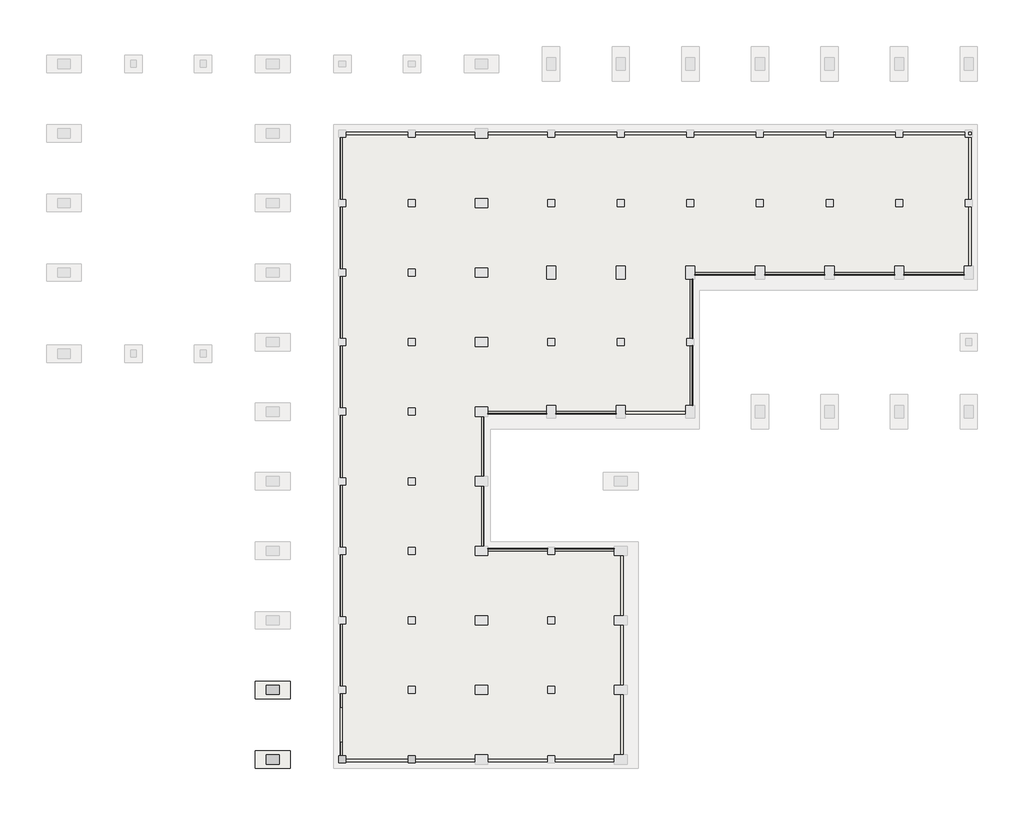
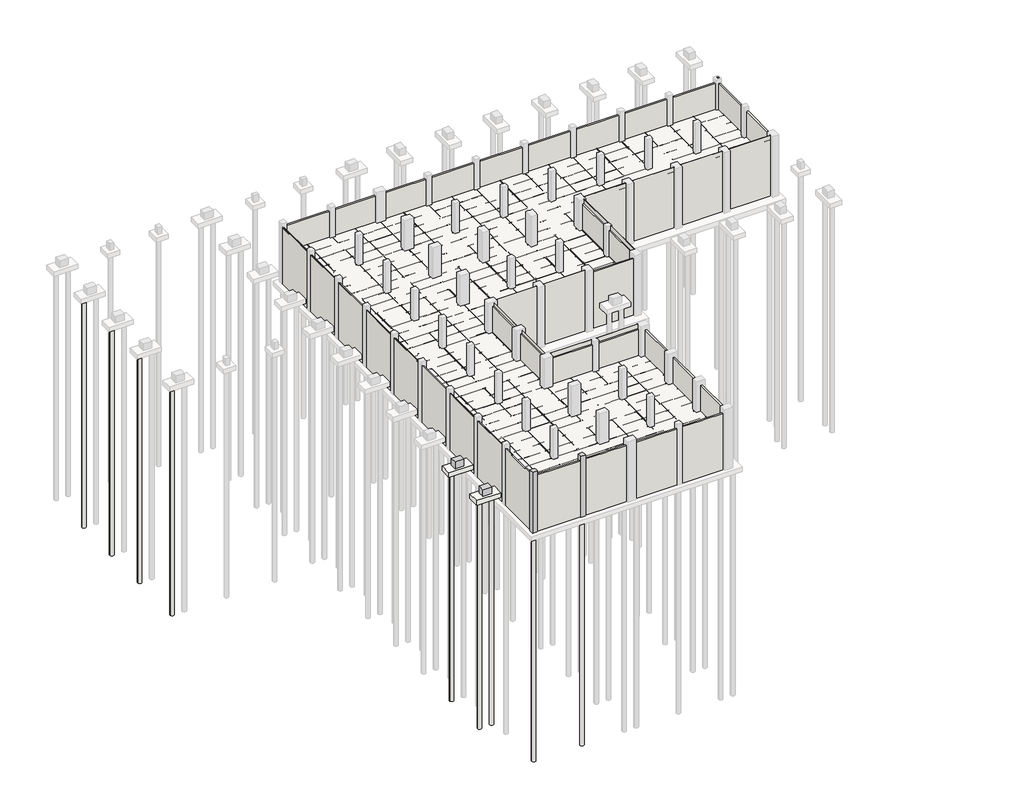
# Not in any storey, part 1 of 16: 12 slabs, 10 walls, 8 beams, 4 columns.
"""IFC4 building model written with IfcOpenShell, lengths in millimetres."""

import ifcopenshell
import ifcopenshell.guid

model = None  # the IFC model being written
_history = None  # IfcOwnerHistory: only IFC2X3 demands one
_inside = {}  # id of a spatial element -> (the spatial element, [elements in it])
_under = {}  # id of a project, library or spatial element -> (it, [spatial elements below it])
_declared = {}  # id of a project -> (the project, [libraries it declares])
_typed = {}  # id of a type object -> (the type object, [elements of that type])
_made_of = {}  # id of a material, layer set ... -> (it, [elements and type objects made of it])


def new_model(schema):
    """Start an empty IFC model of exactly this schema.

    Asked for "IFC4X3", IfcOpenShell would pick the latest addendum, in which some entities
    have other attributes; the version numbers below select the first issue.
    IFC2X3 requires an IfcOwnerHistory on every rooted entity: one is made here for all.
    """
    global model, _history
    if schema == "IFC4X3":
        model = ifcopenshell.file(schema_version=(4, 3, 0, 0))
    else:
        model = ifcopenshell.file(schema=schema)
    _inside.clear()
    _under.clear()
    _declared.clear()
    _typed.clear()
    _made_of.clear()
    _history = None
    if model.schema == "IFC2X3":
        org = make("IfcOrganization", Name="unknown")
        user = make(
            "IfcPersonAndOrganization",
            ThePerson=make("IfcPerson", FamilyName="unknown"),
            TheOrganization=org,
        )
        app = make(
            "IfcApplication",
            ApplicationDeveloper=org,
            Version="unknown",
            ApplicationFullName="unknown",
            ApplicationIdentifier="unknown",
        )
        _history = make(
            "IfcOwnerHistory",
            OwningUser=user,
            OwningApplication=app,
            ChangeAction="ADDED",
            CreationDate=0,
        )
    return model


def make(cls, **values):
    """One entity of the class cls with the attributes given. An attribute that is None is left unset."""
    return model.create_entity(
        cls, **{name: value for name, value in values.items() if value is not None}
    )


def rooted(cls, **values):
    """An entity with a GlobalId (a new one), such as an element, a storey or a relation."""
    return make(cls, GlobalId=ifcopenshell.guid.new(), OwnerHistory=_history, **values)


def si_unit(unit_type, name, prefix=None):
    """IfcSIUnit, for example si_unit("LENGTHUNIT", "METRE", prefix="MILLI")."""
    return make("IfcSIUnit", UnitType=unit_type, Prefix=prefix, Name=name)


def assignment(units):
    """IfcUnitAssignment: the units of a project."""
    return None if units is None else make("IfcUnitAssignment", Units=units)


def point(xyz):
    """IfcCartesianPoint."""
    return None if xyz is None else make("IfcCartesianPoint", Coordinates=xyz)


def direction(xyz):
    """IfcDirection."""
    return None if xyz is None else make("IfcDirection", DirectionRatios=xyz)


def frame(location, z_axis=None, x_axis=None):
    """IfcAxis2Placement3D, a coordinate frame: its origin and axes. An axis left out is left unset."""
    return make(
        "IfcAxis2Placement3D",
        Location=point(location),
        Axis=direction(z_axis),
        RefDirection=direction(x_axis),
    )


def frame_2d(location, x_axis=None):
    """IfcAxis2Placement2D, a coordinate frame in the plane: its origin and x axis."""
    return make(
        "IfcAxis2Placement2D", Location=point(location), RefDirection=direction(x_axis)
    )


def origin():
    """The frame at (0, 0, 0) with its axes left unset."""
    return frame((0.0, 0.0, 0.0))


def place(relative_to, where):
    """IfcLocalPlacement: puts the frame where relative to a parent placement (None: the world)."""
    return make(
        "IfcLocalPlacement", PlacementRelTo=relative_to, RelativePlacement=where
    )


def context(
    kind, dimensions, precision=None, world=None, true_north=None, identifier=None
):
    """IfcGeometricRepresentationContext, for example the 3D "Model" context."""
    return make(
        "IfcGeometricRepresentationContext",
        ContextIdentifier=identifier,
        ContextType=kind,
        CoordinateSpaceDimension=dimensions,
        Precision=precision,
        WorldCoordinateSystem=world,
        TrueNorth=true_north,
    )


def project(units=None, contexts=None):
    """IfcProject with its units and contexts."""
    return rooted(
        "IfcProject",
        Name="project",
        RepresentationContexts=contexts,
        UnitsInContext=assignment(units),
    )


def spatial(cls, under=None, at=None, **own):
    """A site, building, storey or space (cls), placed at a placement, below another one or the project."""
    s = rooted(cls, ObjectPlacement=at, **own)
    if under is not None:
        _under.setdefault(under.id(), (under, []))[1].append(s)
    return s


def polyline(points):
    """IfcPolyline through the points."""
    return make("IfcPolyline", Points=[point(p) for p in points])


def circle_curve(where, radius):
    """IfcCircle in the frame where."""
    return make("IfcCircle", Position=where, Radius=radius)


def trimmed(basis, trim1, trim2, sense, master):
    """IfcTrimmedCurve: the piece of a basis curve between two trims."""
    return make(
        "IfcTrimmedCurve",
        BasisCurve=basis,
        Trim1=trim1,
        Trim2=trim2,
        SenseAgreement=sense,
        MasterRepresentation=master,
    )


def segment(curve, same_sense, transition):
    """IfcCompositeCurveSegment."""
    return make(
        "IfcCompositeCurveSegment",
        Transition=transition,
        SameSense=same_sense,
        ParentCurve=curve,
    )


def composite_curve(segments, self_intersect=None):
    """IfcCompositeCurve: segments joined end to end."""
    return make("IfcCompositeCurve", Segments=segments, SelfIntersect=self_intersect)


def outline(outer, holes=None, kind="AREA"):
    """IfcArbitraryClosedProfileDef: a profile drawn as a closed curve; with holes, ...WithVoids."""
    if holes is None:
        return make("IfcArbitraryClosedProfileDef", ProfileType=kind, OuterCurve=outer)
    return make(
        "IfcArbitraryProfileDefWithVoids",
        ProfileType=kind,
        OuterCurve=outer,
        InnerCurves=holes,
    )


def extrude(swept, where, along, depth):
    """IfcExtrudedAreaSolid: the profile swept, set in the frame where, extruded along a direction by depth."""
    return make(
        "IfcExtrudedAreaSolid",
        SweptArea=swept,
        Position=where,
        ExtrudedDirection=direction(along),
        Depth=depth,
    )


def faces_of(points, faces, orient=None, outer=None):
    """IfcFace entities. A face is a list of loops; a loop is a list of indices into points, from 0.

    orient and outer hold one flag for each loop. By default every Orientation is true, the
    first loop of a face is its IfcFaceOuterBound and the others are IfcFaceBound.
    """
    made = []
    for i, loops in enumerate(faces):
        bounds = []
        for j, loop in enumerate(loops):
            is_outer = j == 0 if outer is None else outer[i][j]
            bounds.append(
                make(
                    "IfcFaceOuterBound" if is_outer else "IfcFaceBound",
                    Bound=make("IfcPolyLoop", Polygon=[points[k] for k in loop]),
                    Orientation=True if orient is None else orient[i][j],
                )
            )
        made.append(make("IfcFace", Bounds=bounds))
    return made


def faceted_brep(points, faces, orient=None, outer=None, voids=None):
    """IfcFacetedBrep: a solid bounded by flat faces; with voids (closed shells), ...WithVoids."""
    shared = [point(p) for p in points]
    hull = make("IfcClosedShell", CfsFaces=faces_of(shared, faces, orient, outer))
    if voids is None:
        return make("IfcFacetedBrep", Outer=hull)
    return make(
        "IfcFacetedBrepWithVoids",
        Outer=hull,
        Voids=[
            make(cls, CfsFaces=faces_of(shared, fs, o, b)) for cls, fs, o, b in voids
        ],
    )


def shape(context_of_items, identifier, shape_type, items):
    """IfcShapeRepresentation: the items that make up one representation, for example the "Body"."""
    return make(
        "IfcShapeRepresentation",
        ContextOfItems=context_of_items,
        RepresentationIdentifier=identifier,
        RepresentationType=shape_type,
        Items=items,
    )


def made_of(thing, what):
    """Note that an element or type object is made of a material, layer set ...; save() writes the relation."""
    if what is not None:
        _made_of.setdefault(what.id(), (what, []))[1].append(thing)
    return thing


def element(
    cls,
    number,
    at=None,
    inside=None,
    cuts=None,
    type_object=None,
    material=None,
    context=None,
    identifier="Body",
    shape_type=None,
    held_by="IfcProductDefinitionShape",
    body=None,
    shapes=None,
    **own,
):
    """One element of the class cls, such as IfcWall. Its Tag is "e" and its number.

    at: its placement. inside: the storey or other place that contains it. cuts: it is an
    opening in that element (IfcRelVoidsElement). A single representation is given by context,
    identifier, shape_type and body (its items); several are given by shapes. held_by: the class
    of the entity that holds the representations. save() writes the other relations.
    """
    e = rooted(cls, Tag="e%d" % number, ObjectPlacement=at, **own)
    if body is not None:
        shapes = [shape(context, identifier, shape_type, body)]
    if shapes is not None:
        e.Representation = make(held_by, Representations=shapes)
    if inside is not None:
        _inside.setdefault(inside.id(), (inside, []))[1].append(e)
    if cuts is not None:
        rooted(
            "IfcRelVoidsElement", RelatingBuildingElement=cuts, RelatedOpeningElement=e
        )
    if type_object is not None:
        _typed.setdefault(type_object.id(), (type_object, []))[1].append(e)
    return made_of(e, material)


def aggregate(whole, parts):
    """IfcRelAggregates: a whole, such as a stair, and the parts it consists of."""
    return rooted("IfcRelAggregates", RelatingObject=whole, RelatedObjects=parts)


def save(model, path):
    """Write the relations noted so far, then the file.

    IfcRelAggregates (storeys below a building ...), IfcRelContainedInSpatialStructure (elements
    in a storey), IfcRelDefinesByType, IfcRelAssociatesMaterial and IfcRelDeclares: one each for
    every whole, place, type object, material and project.
    """
    for whole, parts in _under.values():
        aggregate(whole, parts)
    for where, things in _inside.values():
        rooted(
            "IfcRelContainedInSpatialStructure",
            RelatedElements=things,
            RelatingStructure=where,
        )
    for kind, things in _typed.values():
        rooted("IfcRelDefinesByType", RelatedObjects=things, RelatingType=kind)
    for what, things in _made_of.values():
        rooted("IfcRelAssociatesMaterial", RelatedObjects=things, RelatingMaterial=what)
    for by, libraries in _declared.values():
        rooted("IfcRelDeclares", RelatingContext=by, RelatedDefinitions=libraries)
    model.write(path)


model = new_model("IFC4")

# Units and contexts
model_context = context("Model", 3, world=origin())
ifc_project = project(units=[si_unit("LENGTHUNIT", "METRE", prefix="MILLI")], contexts=[model_context])

# Site, building
site = spatial("IfcSite", under=ifc_project)
building = spatial("IfcBuilding", under=site)

# Beams
placement = place(None, origin())
element("IfcBeam", 1, at=placement, inside=building, context=model_context, shape_type="SweptSolid", body=[
    extrude(outline(composite_curve([segment(polyline([(-4187.0381366, 29900.0), (-4200.0381366, 29900.0), (-4200.0381366, 30100.0), (-4187.0381366, 30100.0), (-4187.0381366, 30020.0)]), True, "CONTINUOUS"), segment(trimmed(circle_curve(frame_2d((-4171.0381366, 30020.0)), 16.0), [point((-4187.0381366, 30020.0))], [point((-4171.0381366, 30004.0))], True, "CARTESIAN"), True, "CONTINUOUS"), segment(polyline([(-4171.0381366, 30004.0), (-3829.0381366, 30004.0)]), True, "CONTINUOUS"), segment(trimmed(circle_curve(frame_2d((-3829.0381366, 30020.0)), 16.0), [point((-3829.0381366, 30004.0))], [point((-3813.0381366, 30020.0))], True, "CARTESIAN"), True, "CONTINUOUS"), segment(polyline([(-3813.0381366, 30020.0), (-3813.0381366, 30100.0), (-3800.0381366, 30100.0), (-3800.0381366, 29900.0), (-3813.0381366, 29900.0), (-3813.0381366, 29980.0)]), True, "CONTINUOUS"), segment(trimmed(circle_curve(frame_2d((-3829.0381366, 29980.0)), 16.0), [point((-3813.0381366, 29980.0))], [point((-3829.0381366, 29996.0))], True, "CARTESIAN"), True, "CONTINUOUS"), segment(polyline([(-3829.0381366, 29996.0), (-4171.0381366, 29996.0)]), True, "CONTINUOUS"), segment(trimmed(circle_curve(frame_2d((-4171.0381366, 29980.0)), 16.0), [point((-4171.0381366, 29996.0))], [point((-4187.0381366, 29980.0))], True, "CARTESIAN"), True, "CONTINUOUS"), segment(polyline([(-4187.0381366, 29980.0), (-4187.0381366, 29900.0)]), True, "CONTINUOUS")], self_intersect=False)), frame((0.0, -59687.3, 0.0), z_axis=(0.0, 1.0, 0.0), x_axis=(0.0, 0.0, 1.0)), (0.0, 0.0, 1.0), 5374.6),
])
element("IfcBeam", 2, at=placement, inside=building, context=model_context, shape_type="SweptSolid", body=[
    extrude(outline(composite_curve([segment(polyline([(-4187.0381366, 26900.0), (-4200.0381366, 26900.0), (-4200.0381366, 27100.0), (-4187.0381366, 27100.0), (-4187.0381366, 27020.0)]), True, "CONTINUOUS"), segment(trimmed(circle_curve(frame_2d((-4171.0381366, 27020.0)), 16.0), [point((-4187.0381366, 27020.0))], [point((-4171.0381366, 27004.0))], True, "CARTESIAN"), True, "CONTINUOUS"), segment(polyline([(-4171.0381366, 27004.0), (-3829.0381366, 27004.0)]), True, "CONTINUOUS"), segment(trimmed(circle_curve(frame_2d((-3829.0381366, 27020.0)), 16.0), [point((-3829.0381366, 27004.0))], [point((-3813.0381366, 27020.0))], True, "CARTESIAN"), True, "CONTINUOUS"), segment(polyline([(-3813.0381366, 27020.0), (-3813.0381366, 27100.0), (-3800.0381366, 27100.0), (-3800.0381366, 26900.0), (-3813.0381366, 26900.0), (-3813.0381366, 26980.0)]), True, "CONTINUOUS"), segment(trimmed(circle_curve(frame_2d((-3829.0381366, 26980.0)), 16.0), [point((-3813.0381366, 26980.0))], [point((-3829.0381366, 26996.0))], True, "CARTESIAN"), True, "CONTINUOUS"), segment(polyline([(-3829.0381366, 26996.0), (-4171.0381366, 26996.0)]), True, "CONTINUOUS"), segment(trimmed(circle_curve(frame_2d((-4171.0381366, 26980.0)), 16.0), [point((-4171.0381366, 26996.0))], [point((-4187.0381366, 26980.0))], True, "CARTESIAN"), True, "CONTINUOUS"), segment(polyline([(-4187.0381366, 26980.0), (-4187.0381366, 26900.0)]), True, "CONTINUOUS")], self_intersect=False)), frame((0.0, -60000.0, 0.0), z_axis=(0.0, 1.0, 0.0), x_axis=(0.0, 0.0, 1.0)), (0.0, 0.0, 1.0), 5887.3),
])
element("IfcBeam", 3, at=placement, inside=building, context=model_context, shape_type="SweptSolid", body=[
    extrude(outline(composite_curve([segment(polyline([(-56977.2, -3800.0381366), (-56977.2, -3950.0381366), (-57052.2, -3950.0381366)]), True, "CONTINUOUS"), segment(trimmed(circle_curve(frame_2d((-57042.2, -3950.0381366)), 10.0), [point((-57052.2, -3950.0381366))], [point((-57042.2, -3940.0381366))], False, "CARTESIAN"), True, "CONTINUOUS"), segment(polyline([(-57042.2, -3940.0381366), (-56983.7, -3930.7726469), (-56983.7, -3819.3036264), (-57042.2, -3810.0381366)]), True, "CONTINUOUS"), segment(trimmed(circle_curve(frame_2d((-57042.2, -3800.0381366)), 10.0), [point((-57042.2, -3810.0381366))], [point((-57052.2, -3800.0381366))], False, "CARTESIAN"), True, "CONTINUOUS"), segment(polyline([(-57052.2, -3800.0381366), (-56977.2, -3800.0381366)]), True, "CONTINUOUS")], self_intersect=False)), frame((24000.0, 0.0, 0.0), z_axis=(1.0, 0.0, 0.0), x_axis=(0.0, 1.0, 0.0)), (0.0, 0.0, 1.0), 2887.3),
])
element("IfcBeam", 4, at=placement, inside=building, context=model_context, shape_type="SweptSolid", body=[
    extrude(outline(composite_curve([segment(polyline([(-58477.2, -3800.0381366), (-58477.2, -3950.0381366), (-58552.2, -3950.0381366)]), True, "CONTINUOUS"), segment(trimmed(circle_curve(frame_2d((-58542.2, -3950.0381366)), 10.0), [point((-58552.2, -3950.0381366))], [point((-58542.2, -3940.0381366))], False, "CARTESIAN"), True, "CONTINUOUS"), segment(polyline([(-58542.2, -3940.0381366), (-58483.7, -3930.7726469), (-58483.7, -3819.3036264), (-58542.2, -3810.0381366)]), True, "CONTINUOUS"), segment(trimmed(circle_curve(frame_2d((-58542.2, -3800.0381366)), 10.0), [point((-58542.2, -3810.0381366))], [point((-58552.2, -3800.0381366))], False, "CARTESIAN"), True, "CONTINUOUS"), segment(polyline([(-58552.2, -3800.0381366), (-58477.2, -3800.0381366)]), True, "CONTINUOUS")], self_intersect=False)), frame((24000.0, 0.0, 0.0), z_axis=(1.0, 0.0, 0.0), x_axis=(0.0, 1.0, 0.0)), (0.0, 0.0, 1.0), 2887.3),
])
element("IfcBeam", 5, at=placement, inside=building, context=model_context, shape_type="SweptSolid", body=[
    extrude(outline(composite_curve([segment(polyline([(-56977.2, -3800.0381366), (-56977.2, -3950.0381366), (-57052.2, -3950.0381366)]), True, "CONTINUOUS"), segment(trimmed(circle_curve(frame_2d((-57042.2, -3950.0381366)), 10.0), [point((-57052.2, -3950.0381366))], [point((-57042.2, -3940.0381366))], False, "CARTESIAN"), True, "CONTINUOUS"), segment(polyline([(-57042.2, -3940.0381366), (-56983.7, -3930.7726469), (-56983.7, -3819.3036264), (-57042.2, -3810.0381366)]), True, "CONTINUOUS"), segment(trimmed(circle_curve(frame_2d((-57042.2, -3800.0381366)), 10.0), [point((-57042.2, -3810.0381366))], [point((-57052.2, -3800.0381366))], False, "CARTESIAN"), True, "CONTINUOUS"), segment(polyline([(-57052.2, -3800.0381366), (-56977.2, -3800.0381366)]), True, "CONTINUOUS")], self_intersect=False)), frame((27112.7, 0.0, 0.0), z_axis=(1.0, 0.0, 0.0), x_axis=(0.0, 1.0, 0.0)), (0.0, 0.0, 1.0), 2774.6),
])
element("IfcBeam", 6, at=placement, inside=building, context=model_context, shape_type="SweptSolid", body=[
    extrude(outline(composite_curve([segment(polyline([(-58477.2, -3800.0381366), (-58477.2, -3950.0381366), (-58552.2, -3950.0381366)]), True, "CONTINUOUS"), segment(trimmed(circle_curve(frame_2d((-58542.2, -3950.0381366)), 10.0), [point((-58552.2, -3950.0381366))], [point((-58542.2, -3940.0381366))], False, "CARTESIAN"), True, "CONTINUOUS"), segment(polyline([(-58542.2, -3940.0381366), (-58483.7, -3930.7726469), (-58483.7, -3819.3036264), (-58542.2, -3810.0381366)]), True, "CONTINUOUS"), segment(trimmed(circle_curve(frame_2d((-58542.2, -3800.0381366)), 10.0), [point((-58542.2, -3810.0381366))], [point((-58552.2, -3800.0381366))], False, "CARTESIAN"), True, "CONTINUOUS"), segment(polyline([(-58552.2, -3800.0381366), (-58477.2, -3800.0381366)]), True, "CONTINUOUS")], self_intersect=False)), frame((27112.7, 0.0, 0.0), z_axis=(1.0, 0.0, 0.0), x_axis=(0.0, 1.0, 0.0)), (0.0, 0.0, 1.0), 2774.6),
])
element("IfcBeam", 7, at=placement, inside=building, context=model_context, shape_type="SweptSolid", body=[
    extrude(outline(composite_curve([segment(polyline([(-56977.2, -3800.0381366), (-56977.2, -3950.0381366), (-57052.2, -3950.0381366)]), True, "CONTINUOUS"), segment(trimmed(circle_curve(frame_2d((-57042.2, -3950.0381366)), 10.0), [point((-57052.2, -3950.0381366))], [point((-57042.2, -3940.0381366))], False, "CARTESIAN"), True, "CONTINUOUS"), segment(polyline([(-57042.2, -3940.0381366), (-56983.7, -3930.7726469), (-56983.7, -3819.3036264), (-57042.2, -3810.0381366)]), True, "CONTINUOUS"), segment(trimmed(circle_curve(frame_2d((-57042.2, -3800.0381366)), 10.0), [point((-57042.2, -3810.0381366))], [point((-57052.2, -3800.0381366))], False, "CARTESIAN"), True, "CONTINUOUS"), segment(polyline([(-57052.2, -3800.0381366), (-56977.2, -3800.0381366)]), True, "CONTINUOUS")], self_intersect=False)), frame((30112.7, 0.0, 0.0), z_axis=(1.0, 0.0, 0.0), x_axis=(0.0, 1.0, 0.0)), (0.0, 0.0, 1.0), 2774.6),
])
element("IfcBeam", 8, at=placement, inside=building, context=model_context, shape_type="SweptSolid", body=[
    extrude(outline(composite_curve([segment(polyline([(-58477.2, -3800.0381366), (-58477.2, -3950.0381366), (-58552.2, -3950.0381366)]), True, "CONTINUOUS"), segment(trimmed(circle_curve(frame_2d((-58542.2, -3950.0381366)), 10.0), [point((-58552.2, -3950.0381366))], [point((-58542.2, -3940.0381366))], False, "CARTESIAN"), True, "CONTINUOUS"), segment(polyline([(-58542.2, -3940.0381366), (-58483.7, -3930.7726469), (-58483.7, -3819.3036264), (-58542.2, -3810.0381366)]), True, "CONTINUOUS"), segment(trimmed(circle_curve(frame_2d((-58542.2, -3800.0381366)), 10.0), [point((-58542.2, -3810.0381366))], [point((-58552.2, -3800.0381366))], False, "CARTESIAN"), True, "CONTINUOUS"), segment(polyline([(-58552.2, -3800.0381366), (-58477.2, -3800.0381366)]), True, "CONTINUOUS")], self_intersect=False)), frame((30112.7, 0.0, 0.0), z_axis=(1.0, 0.0, 0.0), x_axis=(0.0, 1.0, 0.0)), (0.0, 0.0, 1.0), 2774.6),
])

# Columns
element("IfcColumn", 9, ObjectType="RC_Column_Rectangular", at=placement, inside=building, context=model_context, shape_type="Brep", body=[
    faceted_brep([(17450.0, -53600.0, -700.0381366), (18550.0, -53600.0, -700.0381366), (18550.0, -54400.0, -700.0381366), (17450.0, -54400.0, -700.0381366), (17450.0, -53600.0, 199.9618634), (17800.0, -53600.0, 199.9618634), (18200.0, -53600.0, 199.9618634), (18550.0, -53600.0, 199.9618634), (18550.0, -53600.0, -0.0381366), (18550.0, -54400.0, 199.9618634), (18550.0, -54400.0, -0.0381366), (18200.0, -54400.0, 199.9618634), (17800.0, -54400.0, 199.9618634), (17450.0, -54400.0, 199.9618634)], [[[0, 1, 2, 3]], [[4, 5, 6, 7, 8, 1, 0]], [[7, 9, 10, 2, 1, 8]], [[9, 11, 12, 13, 3, 2, 10]], [[13, 4, 0, 3]], [[4, 13, 12, 11, 9, 7, 6, 5]]]),
])
element("IfcColumn", 10, ObjectType="RC_Column_Rectangular", at=placement, inside=building, context=model_context, shape_type="Brep", body=[
    faceted_brep([(17450.0, -59600.0, -700.0381366), (18550.0, -59600.0, -700.0381366), (18550.0, -60400.0, -700.0381366), (17450.0, -60400.0, -700.0381366), (17450.0, -59600.0, 199.9618634), (18200.0, -59600.0, 199.9618634), (18550.0, -59600.0, 199.9618634), (18550.0, -59600.0, -0.0381366), (18550.0, -59800.0, 199.9618634), (18550.0, -60400.0, 199.9618634), (17450.0, -60400.0, 199.9618634)], [[[0, 1, 2, 3]], [[4, 5, 6, 7, 1, 0]], [[6, 8, 9, 2, 1, 7]], [[9, 10, 3, 2]], [[10, 4, 0, 3]], [[4, 10, 9, 8, 6, 5]]]),
])
element("IfcColumn", 11, ObjectType="RC_Column_Rectangular", at=placement, inside=building, context=model_context, shape_type="Brep", body=[
    faceted_brep([(30300.0, -59700.0, -7800.0381366), (30300.0, -60000.0, -7800.0381366), (30300.0, -60200.0, -7800.0381366), (30300.0, -60300.0, -7800.0381366), (29700.0, -60300.0, -7800.0381366), (29700.0, -60200.0, -7800.0381366), (29700.0, -60000.0, -7800.0381366), (29700.0, -59700.0, -7800.0381366), (30300.0, -59700.0, 199.9618634), (30300.0, -60000.0, 199.9618634), (30300.0, -60200.0, 199.9618634), (30300.0, -60300.0, 199.9618634), (30300.0, -59700.0, -3832.0381366), (30300.0, -59700.0, -3800.0381366), (30300.0, -59700.0, -0.0381366), (29700.0, -60300.0, 199.9618634), (29700.0, -60200.0, 199.9618634), (29700.0, -60000.0, 199.9618634), (29700.0, -59700.0, 199.9618634), (29700.0, -59700.0, -0.0381366), (29700.0, -59700.0, -3800.0381366), (29700.0, -59700.0, -3832.0381366), (29825.0, -59700.0, 199.9618634), (30175.0, -59700.0, 199.9618634)], [[[0, 1, 2, 3, 4, 5, 6, 7]], [[8, 9, 10, 11, 3, 2, 1, 0, 12, 13, 14]], [[11, 15, 4, 3]], [[15, 16, 17, 18, 19, 20, 21, 7, 6, 5, 4]], [[18, 22, 23, 8, 14, 13, 12, 0, 7, 21, 20, 19]], [[8, 23, 22, 18, 17, 16, 15, 11, 10, 9]]]),
])
element("IfcColumn", 12, ObjectType="RC_Column_Rectangular", at=placement, inside=building, context=model_context, shape_type="Brep", body=[
    faceted_brep([(24300.0, -59700.0, -7800.0381366), (24300.0, -60000.0, -7800.0381366), (24300.0, -60200.0, -7800.0381366), (24300.0, -60300.0, -7800.0381366), (23700.0, -60300.0, -7800.0381366), (23700.0, -59700.0, -7800.0381366), (23800.0, -59700.0, -7800.0381366), (24000.0, -59700.0, -7800.0381366), (24300.0, -59700.0, 199.9618634), (24300.0, -60000.0, 199.9618634), (24300.0, -60200.0, 199.9618634), (24300.0, -60300.0, 199.9618634), (24300.0, -59700.0, -3832.0381366), (24300.0, -59700.0, -3800.0381366), (24300.0, -59700.0, -0.0381366), (23700.0, -60300.0, 199.9618634), (23700.0, -60200.0, 199.9618634), (23700.0, -59800.0, 199.9618634), (23700.0, -59700.0, 199.9618634), (23700.0, -59700.0, -0.0381366), (24000.0, -59700.0, 199.9618634)], [[[0, 1, 2, 3, 4, 5, 6, 7]], [[8, 9, 10, 11, 3, 2, 1, 0, 12, 13, 14]], [[11, 15, 4, 3]], [[15, 16, 17, 18, 19, 5, 4]], [[18, 20, 8, 14, 13, 12, 0, 7, 6, 5, 19]], [[8, 20, 18, 17, 16, 15, 11, 10, 9]]]),
])

# Slabs
element("IfcSlab", 13, at=placement, inside=building, context=model_context, shape_type="SweptSolid", body=[
    extrude(outline(polyline([(36550.0, -59600.0), (35450.0, -59600.0), (35450.0, -60000.0), (30300.0, -60000.0), (30300.0, -59700.0), (29700.0, -59700.0), (29700.0, -60000.0), (24300.0, -60000.0), (24300.0, -59700.0), (24000.0, -59700.0), (24000.0, -54300.0), (24300.0, -54300.0), (24300.0, -53700.0), (24000.0, -53700.0), (24000.0, -48300.0), (24300.0, -48300.0), (24300.0, -47700.0), (24000.0, -47700.0), (24000.0, -42300.0), (24300.0, -42300.0), (24300.0, -41700.0), (24000.0, -41700.0), (24000.0, -36300.0), (24300.0, -36300.0), (24300.0, -35700.0), (24000.0, -35700.0), (24000.0, -30300.0), (24300.0, -30300.0), (24300.0, -29700.0), (24000.0, -29700.0), (24000.0, -24300.0), (24300.0, -24300.0), (24300.0, -23700.0), (24000.0, -23700.0), (24000.0, -18300.0), (24300.0, -18300.0), (24300.0, -17700.0), (24000.0, -17700.0), (24000.0, -12300.0), (24300.0, -12300.0), (24300.0, -11700.0), (24000.0, -11700.0), (24000.0, -6300.0), (24300.0, -6300.0), (24300.0, -6000.0), (29700.0, -6000.0), (29700.0, -6300.0), (30300.0, -6300.0), (30300.0, -6000.0), (35450.0, -6000.0), (35450.0, -6400.0), (36550.0, -6400.0), (36550.0, -6000.0), (41700.0, -6000.0), (41700.0, -6300.0), (42300.0, -6300.0), (42300.0, -6000.0), (47700.0, -6000.0), (47700.0, -6300.0), (48300.0, -6300.0), (48300.0, -6000.0), (53700.0, -6000.0), (53700.0, -6300.0), (54300.0, -6300.0), (54300.0, -6000.0), (59700.0, -6000.0), (59700.0, -6300.0), (60300.0, -6300.0), (60300.0, -6000.0), (65700.0, -6000.0), (65700.0, -6300.0), (66300.0, -6300.0), (66300.0, -6000.0), (71700.0, -6000.0), (71700.0, -6300.0), (72300.0, -6300.0), (72300.0, -6000.0), (77700.0, -6000.0), (77700.0, -6300.0), (78000.0, -6300.0), (78000.0, -11700.0), (77700.0, -11700.0), (77700.0, -12300.0), (78000.0, -12300.0), (78000.0, -17450.0), (77600.0, -17450.0), (77600.0, -18000.0), (72400.0, -18000.0), (72400.0, -17450.0), (71600.0, -17450.0), (71600.0, -18000.0), (66400.0, -18000.0), (66400.0, -17450.0), (65600.0, -17450.0), (65600.0, -18000.0), (60400.0, -18000.0), (60400.0, -17450.0), (59600.0, -17450.0), (59600.0, -18000.0), (54400.0, -18000.0), (54400.0, -17450.0), (53600.0, -17450.0), (53600.0, -18550.0), (54000.0, -18550.0), (54000.0, -23700.0), (53700.0, -23700.0), (53700.0, -24300.0), (54000.0, -24300.0), (54000.0, -29450.0), (53600.0, -29450.0), (53600.0, -30000.0), (48400.0, -30000.0), (48400.0, -29450.0), (47600.0, -29450.0), (47600.0, -30000.0), (42400.0, -30000.0), (42400.0, -29450.0), (41600.0, -29450.0), (41600.0, -30000.0), (36550.0, -30000.0), (36550.0, -29600.0), (35450.0, -29600.0), (35450.0, -30400.0), (36000.0, -30400.0), (36000.0, -35600.0), (35450.0, -35600.0), (35450.0, -36400.0), (36000.0, -36400.0), (36000.0, -41600.0), (35450.0, -41600.0), (35450.0, -42400.0), (36550.0, -42400.0), (36550.0, -42000.0), (41700.0, -42000.0), (41700.0, -42300.0), (42300.0, -42300.0), (42300.0, -42000.0), (47450.0, -42000.0), (47450.0, -42400.0), (48000.0, -42400.0), (48000.0, -47600.0), (47450.0, -47600.0), (47450.0, -48400.0), (48000.0, -48400.0), (48000.0, -53600.0), (47450.0, -53600.0), (47450.0, -54400.0), (48000.0, -54400.0), (48000.0, -59600.0), (47450.0, -59600.0), (47450.0, -60000.0), (42300.0, -60000.0), (42300.0, -59700.0), (41700.0, -59700.0), (41700.0, -60000.0), (36550.0, -60000.0), (36550.0, -59600.0)]), holes=[polyline([(36550.0, -53600.0), (35450.0, -53600.0), (35450.0, -54400.0), (36550.0, -54400.0), (36550.0, -53600.0)]), polyline([(36550.0, -47600.0), (35450.0, -47600.0), (35450.0, -48400.0), (36550.0, -48400.0), (36550.0, -47600.0)]), polyline([(36550.0, -23600.0), (35450.0, -23600.0), (35450.0, -24400.0), (36550.0, -24400.0), (36550.0, -23600.0)]), polyline([(36550.0, -17600.0), (35450.0, -17600.0), (35450.0, -18400.0), (36550.0, -18400.0), (36550.0, -17600.0)]), polyline([(36550.0, -11600.0), (35450.0, -11600.0), (35450.0, -12400.0), (36550.0, -12400.0), (36550.0, -11600.0)]), polyline([(42400.0, -18550.0), (42400.0, -17450.0), (41600.0, -17450.0), (41600.0, -18550.0), (42400.0, -18550.0)]), polyline([(48400.0, -18550.0), (48400.0, -17450.0), (47600.0, -17450.0), (47600.0, -18550.0), (48400.0, -18550.0)]), polyline([(30300.0, -12300.0), (30300.0, -11700.0), (29700.0, -11700.0), (29700.0, -12300.0), (30300.0, -12300.0)]), polyline([(42300.0, -12300.0), (42300.0, -11700.0), (41700.0, -11700.0), (41700.0, -12300.0), (42300.0, -12300.0)]), polyline([(48300.0, -12300.0), (48300.0, -11700.0), (47700.0, -11700.0), (47700.0, -12300.0), (48300.0, -12300.0)]), polyline([(54300.0, -12300.0), (54300.0, -11700.0), (53700.0, -11700.0), (53700.0, -12300.0), (54300.0, -12300.0)]), polyline([(60300.0, -12300.0), (60300.0, -11700.0), (59700.0, -11700.0), (59700.0, -12300.0), (60300.0, -12300.0)]), polyline([(66300.0, -12300.0), (66300.0, -11700.0), (65700.0, -11700.0), (65700.0, -12300.0), (66300.0, -12300.0)]), polyline([(72300.0, -12300.0), (72300.0, -11700.0), (71700.0, -11700.0), (71700.0, -12300.0), (72300.0, -12300.0)]), polyline([(30300.0, -24300.0), (30300.0, -23700.0), (29700.0, -23700.0), (29700.0, -24300.0), (30300.0, -24300.0)]), polyline([(42300.0, -24300.0), (42300.0, -23700.0), (41700.0, -23700.0), (41700.0, -24300.0), (42300.0, -24300.0)]), polyline([(48300.0, -24300.0), (48300.0, -23700.0), (47700.0, -23700.0), (47700.0, -24300.0), (48300.0, -24300.0)]), polyline([(30300.0, -18300.0), (30300.0, -17700.0), (29700.0, -17700.0), (29700.0, -18300.0), (30300.0, -18300.0)]), polyline([(30300.0, -30300.0), (30300.0, -29700.0), (29700.0, -29700.0), (29700.0, -30300.0), (30300.0, -30300.0)]), polyline([(30300.0, -36300.0), (30300.0, -35700.0), (29700.0, -35700.0), (29700.0, -36300.0), (30300.0, -36300.0)]), polyline([(30300.0, -42300.0), (30300.0, -41700.0), (29700.0, -41700.0), (29700.0, -42300.0), (30300.0, -42300.0)]), polyline([(30300.0, -48300.0), (30300.0, -47700.0), (29700.0, -47700.0), (29700.0, -48300.0), (30300.0, -48300.0)]), polyline([(30300.0, -54300.0), (30300.0, -53700.0), (29700.0, -53700.0), (29700.0, -54300.0), (30300.0, -54300.0)]), polyline([(42300.0, -48300.0), (42300.0, -47700.0), (41700.0, -47700.0), (41700.0, -48300.0), (42300.0, -48300.0)]), polyline([(42300.0, -54300.0), (42300.0, -53700.0), (41700.0, -53700.0), (41700.0, -54300.0), (42300.0, -54300.0)])]), frame((0.0, 0.0, -3832.0381366), z_axis=(0.0, 0.0, 1.0), x_axis=(1.0, 0.0, 0.0)), (0.0, 0.0, 1.0), 32.0),
])
element("IfcSlab", 14, ObjectType="Foundation Rectangular (Non-Pile)", at=placement, inside=building, context=model_context, shape_type="SweptSolid", body=[
    extrude(outline(polyline([(19500.0, -54750.0), (16500.0, -54750.0), (16500.0, -53250.0), (19500.0, -53250.0), (19500.0, -54750.0)])), frame((0.0, 0.0, -1300.0381366), z_axis=(0.0, 0.0, 1.0), x_axis=(1.0, 0.0, 0.0)), (0.0, 0.0, 1.0), 600.0),
])
element("IfcSlab", 15, ObjectType="Foundation Rectangular (Non-Pile)", at=placement, inside=building, context=model_context, shape_type="SweptSolid", body=[
    extrude(outline(polyline([(19500.0, -60750.0), (16500.0, -60750.0), (16500.0, -59250.0), (19500.0, -59250.0), (19500.0, -60750.0)])), frame((0.0, 0.0, -1300.0381366), z_axis=(0.0, 0.0, 1.0), x_axis=(1.0, 0.0, 0.0)), (0.0, 0.0, 1.0), 600.0),
])
element("IfcSlab", 16, ObjectType="PILE", at=placement, inside=building, context=model_context, shape_type="SweptSolid", body=[
    extrude(outline(composite_curve([segment(trimmed(circle_curve(frame_2d((17250.0, -60000.0)), 250.0), [point((17000.0, -60000.0))], [point((17500.0, -60000.0))], False, "CARTESIAN"), True, "CONTINUOUS"), segment(trimmed(circle_curve(frame_2d((17250.0, -60000.0)), 250.0), [point((17500.0, -60000.0))], [point((17000.0, -60000.0))], False, "CARTESIAN"), True, "CONTINUOUS")], self_intersect=False)), frame((0.0, 0.0, -31300.0381366), z_axis=(0.0, 0.0, 1.0), x_axis=(1.0, 0.0, 0.0)), (0.0, 0.0, 1.0), 30000.0),
])
element("IfcSlab", 17, ObjectType="PILE", at=placement, inside=building, context=model_context, shape_type="SweptSolid", body=[
    extrude(outline(composite_curve([segment(trimmed(circle_curve(frame_2d((18750.0, -60000.0)), 250.0), [point((18500.0, -60000.0))], [point((19000.0, -60000.0))], False, "CARTESIAN"), True, "CONTINUOUS"), segment(trimmed(circle_curve(frame_2d((18750.0, -60000.0)), 250.0), [point((19000.0, -60000.0))], [point((18500.0, -60000.0))], False, "CARTESIAN"), True, "CONTINUOUS")], self_intersect=False)), frame((0.0, 0.0, -31300.0381366), z_axis=(0.0, 0.0, 1.0), x_axis=(1.0, 0.0, 0.0)), (0.0, 0.0, 1.0), 30000.0),
])
element("IfcSlab", 18, ObjectType="PILE", at=placement, inside=building, context=model_context, shape_type="SweptSolid", body=[
    extrude(outline(composite_curve([segment(trimmed(circle_curve(frame_2d((17250.0, -54000.0)), 250.0), [point((17000.0, -54000.0))], [point((17500.0, -54000.0))], False, "CARTESIAN"), True, "CONTINUOUS"), segment(trimmed(circle_curve(frame_2d((17250.0, -54000.0)), 250.0), [point((17500.0, -54000.0))], [point((17000.0, -54000.0))], False, "CARTESIAN"), True, "CONTINUOUS")], self_intersect=False)), frame((0.0, 0.0, -31300.0381366), z_axis=(0.0, 0.0, 1.0), x_axis=(1.0, 0.0, 0.0)), (0.0, 0.0, 1.0), 30000.0),
])
element("IfcSlab", 19, ObjectType="PILE", at=placement, inside=building, context=model_context, shape_type="SweptSolid", body=[
    extrude(outline(composite_curve([segment(trimmed(circle_curve(frame_2d((-750.0, -25000.0)), 250.0), [point((-1000.0, -25000.0))], [point((-500.0, -25000.0))], False, "CARTESIAN"), True, "CONTINUOUS"), segment(trimmed(circle_curve(frame_2d((-750.0, -25000.0)), 250.0), [point((-500.0, -25000.0))], [point((-1000.0, -25000.0))], False, "CARTESIAN"), True, "CONTINUOUS")], self_intersect=False)), frame((0.0, 0.0, -31300.0381366), z_axis=(0.0, 0.0, 1.0), x_axis=(1.0, 0.0, 0.0)), (0.0, 0.0, 1.0), 30000.0),
])
element("IfcSlab", 20, ObjectType="PILE", at=placement, inside=building, context=model_context, shape_type="SweptSolid", body=[
    extrude(outline(composite_curve([segment(trimmed(circle_curve(frame_2d((-750.0, -18000.0)), 250.0), [point((-1000.0, -18000.0))], [point((-500.0, -18000.0))], False, "CARTESIAN"), True, "CONTINUOUS"), segment(trimmed(circle_curve(frame_2d((-750.0, -18000.0)), 250.0), [point((-500.0, -18000.0))], [point((-1000.0, -18000.0))], False, "CARTESIAN"), True, "CONTINUOUS")], self_intersect=False)), frame((0.0, 0.0, -31300.0381366), z_axis=(0.0, 0.0, 1.0), x_axis=(1.0, 0.0, 0.0)), (0.0, 0.0, 1.0), 30000.0),
])
element("IfcSlab", 21, ObjectType="PILE", at=placement, inside=building, context=model_context, shape_type="SweptSolid", body=[
    extrude(outline(composite_curve([segment(trimmed(circle_curve(frame_2d((-750.0, -12000.0)), 250.0), [point((-1000.0, -12000.0))], [point((-500.0, -12000.0))], False, "CARTESIAN"), True, "CONTINUOUS"), segment(trimmed(circle_curve(frame_2d((-750.0, -12000.0)), 250.0), [point((-500.0, -12000.0))], [point((-1000.0, -12000.0))], False, "CARTESIAN"), True, "CONTINUOUS")], self_intersect=False)), frame((0.0, 0.0, -31300.0381366), z_axis=(0.0, 0.0, 1.0), x_axis=(1.0, 0.0, 0.0)), (0.0, 0.0, 1.0), 30000.0),
])
element("IfcSlab", 22, ObjectType="PILE", at=placement, inside=building, context=model_context, shape_type="SweptSolid", body=[
    extrude(outline(composite_curve([segment(trimmed(circle_curve(frame_2d((-750.0, -6000.0)), 250.0), [point((-1000.0, -6000.0))], [point((-500.0, -6000.0))], False, "CARTESIAN"), True, "CONTINUOUS"), segment(trimmed(circle_curve(frame_2d((-750.0, -6000.0)), 250.0), [point((-500.0, -6000.0))], [point((-1000.0, -6000.0))], False, "CARTESIAN"), True, "CONTINUOUS")], self_intersect=False)), frame((0.0, 0.0, -31300.0381366), z_axis=(0.0, 0.0, 1.0), x_axis=(1.0, 0.0, 0.0)), (0.0, 0.0, 1.0), 30000.0),
])
element("IfcSlab", 23, ObjectType="PILE", at=placement, inside=building, context=model_context, shape_type="SweptSolid", body=[
    extrude(outline(composite_curve([segment(trimmed(circle_curve(frame_2d((30000.0, -60000.0)), 250.0), [point((29750.0, -60000.0))], [point((30250.0, -60000.0))], False, "CARTESIAN"), True, "CONTINUOUS"), segment(trimmed(circle_curve(frame_2d((30000.0, -60000.0)), 250.0), [point((30250.0, -60000.0))], [point((29750.0, -60000.0))], False, "CARTESIAN"), True, "CONTINUOUS")], self_intersect=False)), frame((0.0, 0.0, -37950.0381366), z_axis=(0.0, 0.0, 1.0), x_axis=(1.0, 0.0, 0.0)), (0.0, 0.0, 1.0), 29550.0),
])
element("IfcSlab", 24, ObjectType="PILE", at=placement, inside=building, context=model_context, shape_type="SweptSolid", body=[
    extrude(outline(composite_curve([segment(trimmed(circle_curve(frame_2d((24000.0, -60000.0)), 250.0), [point((23750.0, -60000.0))], [point((24250.0, -60000.0))], False, "CARTESIAN"), True, "CONTINUOUS"), segment(trimmed(circle_curve(frame_2d((24000.0, -60000.0)), 250.0), [point((24250.0, -60000.0))], [point((23750.0, -60000.0))], False, "CARTESIAN"), True, "CONTINUOUS")], self_intersect=False)), frame((0.0, 0.0, -37950.0381366), z_axis=(0.0, 0.0, 1.0), x_axis=(1.0, 0.0, 0.0)), (0.0, 0.0, 1.0), 29550.0),
])

# Walls
element("IfcWall", 25, at=placement, inside=building, context=model_context, shape_type="Brep", body=[
    faceted_brep([(24000.0, -6300.0, -7800.0381366), (24000.0, -6300.0, -400.0381366), (24000.0, -11700.0, -400.0381366), (24000.0, -11700.0, -7800.0381366), (23800.0, -6300.0, -300.0381366), (23800.0, -6300.0, -7800.0381366), (23800.0, -11700.0, -7800.0381366), (23800.0, -11700.0, -300.0381366), (23825.0, -6300.0, -300.0381366), (23825.0, -11700.0, -300.0381366), (23825.0, -6300.0, -400.0381366), (23825.0, -11700.0, -400.0381366)], [[[0, 1, 2, 3]], [[4, 5, 6, 7]], [[5, 0, 3, 6]], [[8, 4, 7, 9]], [[1, 10, 11, 2]], [[10, 8, 9, 11]], [[1, 0, 5, 4, 8, 10]], [[3, 2, 11, 9, 7, 6]]]),
    faceted_brep([(24000.0, -12300.0, -7800.0381366), (24000.0, -12300.0, -400.0381366), (24000.0, -17700.0, -400.0381366), (24000.0, -17700.0, -7800.0381366), (23800.0, -12300.0, -300.0381366), (23800.0, -12300.0, -7800.0381366), (23800.0, -17700.0, -7800.0381366), (23800.0, -17700.0, -300.0381366), (23825.0, -12300.0, -300.0381366), (23825.0, -17700.0, -300.0381366), (23825.0, -12300.0, -400.0381366), (23825.0, -17700.0, -400.0381366)], [[[0, 1, 2, 3]], [[4, 5, 6, 7]], [[5, 0, 3, 6]], [[8, 4, 7, 9]], [[1, 10, 11, 2]], [[10, 8, 9, 11]], [[1, 0, 5, 4, 8, 10]], [[3, 2, 11, 9, 7, 6]]]),
    faceted_brep([(24000.0, -24300.0, -7800.0381366), (24000.0, -24300.0, -400.0381366), (24000.0, -29700.0, -400.0381366), (24000.0, -29700.0, -7800.0381366), (23800.0, -24300.0, -300.0381366), (23800.0, -24300.0, -7800.0381366), (23800.0, -29700.0, -7800.0381366), (23800.0, -29700.0, -300.0381366), (23825.0, -24300.0, -300.0381366), (23825.0, -29700.0, -300.0381366), (23825.0, -24300.0, -400.0381366), (23825.0, -29700.0, -400.0381366)], [[[0, 1, 2, 3]], [[4, 5, 6, 7]], [[5, 0, 3, 6]], [[8, 4, 7, 9]], [[1, 10, 11, 2]], [[10, 8, 9, 11]], [[1, 0, 5, 4, 8, 10]], [[3, 2, 11, 9, 7, 6]]]),
    faceted_brep([(24000.0, -23700.0, -400.0381366), (24000.0, -23700.0, -7800.0381366), (24000.0, -18300.0, -7800.0381366), (24000.0, -18300.0, -400.0381366), (23800.0, -23700.0, -7800.0381366), (23800.0, -23700.0, -300.0381366), (23800.0, -18300.0, -300.0381366), (23800.0, -18300.0, -7800.0381366), (23825.0, -23700.0, -300.0381366), (23825.0, -18300.0, -300.0381366), (23825.0, -23700.0, -400.0381366), (23825.0, -18300.0, -400.0381366)], [[[0, 1, 2, 3]], [[4, 5, 6, 7]], [[1, 4, 7, 2]], [[5, 8, 9, 6]], [[10, 0, 3, 11]], [[8, 10, 11, 9]], [[1, 0, 10, 8, 5, 4]], [[3, 2, 7, 6, 9, 11]]]),
    faceted_brep([(24000.0, -30300.0, -7800.0381366), (24000.0, -30300.0, -400.0381366), (24000.0, -35700.0, -400.0381366), (24000.0, -35700.0, -7800.0381366), (23800.0, -30300.0, -300.0381366), (23800.0, -30300.0, -7800.0381366), (23800.0, -35700.0, -7800.0381366), (23800.0, -35700.0, -300.0381366), (23825.0, -30300.0, -300.0381366), (23825.0, -35700.0, -300.0381366), (23825.0, -30300.0, -400.0381366), (23825.0, -35700.0, -400.0381366)], [[[0, 1, 2, 3]], [[4, 5, 6, 7]], [[5, 0, 3, 6]], [[8, 4, 7, 9]], [[1, 10, 11, 2]], [[10, 8, 9, 11]], [[1, 0, 5, 4, 8, 10]], [[3, 2, 11, 9, 7, 6]]]),
    faceted_brep([(24000.0, -36300.0, -7800.0381366), (24000.0, -36300.0, -400.0381366), (24000.0, -41700.0, -400.0381366), (24000.0, -41700.0, -7800.0381366), (23800.0, -36300.0, -300.0381366), (23800.0, -36300.0, -7800.0381366), (23800.0, -41700.0, -7800.0381366), (23800.0, -41700.0, -300.0381366), (23825.0, -36300.0, -300.0381366), (23825.0, -41700.0, -300.0381366), (23825.0, -36300.0, -400.0381366), (23825.0, -41700.0, -400.0381366)], [[[0, 1, 2, 3]], [[4, 5, 6, 7]], [[5, 0, 3, 6]], [[8, 4, 7, 9]], [[1, 10, 11, 2]], [[10, 8, 9, 11]], [[1, 0, 5, 4, 8, 10]], [[3, 2, 11, 9, 7, 6]]]),
    faceted_brep([(24000.0, -42300.0, -7800.0381366), (24000.0, -42300.0, -400.0381366), (24000.0, -47700.0, -400.0381366), (24000.0, -47700.0, -7800.0381366), (23800.0, -42300.0, -300.0381366), (23800.0, -42300.0, -7800.0381366), (23800.0, -47700.0, -7800.0381366), (23800.0, -47700.0, -300.0381366), (23825.0, -42300.0, -300.0381366), (23825.0, -47700.0, -300.0381366), (23825.0, -42300.0, -400.0381366), (23825.0, -47700.0, -400.0381366)], [[[0, 1, 2, 3]], [[4, 5, 6, 7]], [[5, 0, 3, 6]], [[8, 4, 7, 9]], [[1, 10, 11, 2]], [[10, 8, 9, 11]], [[1, 0, 5, 4, 8, 10]], [[3, 2, 11, 9, 7, 6]]]),
    faceted_brep([(24000.0, -48300.0, -7800.0381366), (24000.0, -48300.0, -400.0381366), (24000.0, -53700.0, -400.0381366), (24000.0, -53700.0, -7800.0381366), (23800.0, -48300.0, -300.0381366), (23800.0, -48300.0, -7800.0381366), (23800.0, -53700.0, -7800.0381366), (23800.0, -53700.0, -300.0381366), (23825.0, -48300.0, -300.0381366), (23825.0, -53700.0, -300.0381366), (23825.0, -48300.0, -400.0381366), (23825.0, -53700.0, -400.0381366)], [[[0, 1, 2, 3]], [[4, 5, 6, 7]], [[5, 0, 3, 6]], [[8, 4, 7, 9]], [[1, 10, 11, 2]], [[10, 8, 9, 11]], [[1, 0, 5, 4, 8, 10]], [[3, 2, 11, 9, 7, 6]]]),
    faceted_brep([(24000.0, -54300.0, -7800.0381366), (24000.0, -54300.0, -400.0381366), (24000.0, -55500.0, -400.0381366), (24000.0, -55500.0, -500.0381366), (24000.0, -58500.0, -500.0381366), (24000.0, -58500.0, -400.0381366), (24000.0, -59700.0, -400.0381366), (24000.0, -59700.0, -7800.0381366), (23800.0, -54300.0, -300.0381366), (23800.0, -54300.0, -7800.0381366), (23800.0, -59700.0, -7800.0381366), (23800.0, -59700.0, -300.0381366), (23800.0, -58500.0, -300.0381366), (23800.0, -58500.0, -500.0381366), (23800.0, -55500.0, -500.0381366), (23800.0, -55500.0, -300.0381366), (23825.0, -54300.0, -300.0381366), (23825.0, -55500.0, -300.0381366), (23825.0, -59700.0, -300.0381366), (23825.0, -58500.0, -300.0381366), (23825.0, -54300.0, -400.0381366), (23825.0, -55500.0, -400.0381366), (23825.0, -59700.0, -400.0381366), (23825.0, -58500.0, -400.0381366)], [[[0, 1, 2, 3, 4, 5, 6, 7]], [[8, 9, 10, 11, 12, 13, 14, 15]], [[9, 0, 7, 10]], [[16, 8, 15, 17]], [[11, 18, 19, 12]], [[1, 20, 21, 2]], [[22, 6, 5, 23]], [[20, 16, 17, 21]], [[18, 22, 23, 19]], [[1, 0, 9, 8, 16, 20]], [[7, 6, 22, 18, 11, 10]], [[3, 14, 13, 4]], [[4, 13, 12, 19, 23, 5]], [[14, 3, 2, 21, 17, 15]]]),
])
element("IfcWall", 26, at=placement, inside=building, context=model_context, shape_type="SweptSolid", body=[
    extrude(outline(polyline([(-7800.0381366, 24000.0), (-7800.0381366, 78200.0), (199.9618634, 78200.0), (199.9618634, 78000.0), (-400.0381366, 78000.0), (-400.0381366, 24000.0), (-7800.0381366, 24000.0)])), frame((0.0, -6100.0, 0.0), z_axis=(0.0, 1.0, 0.0), x_axis=(0.0, 0.0, 1.0)), (0.0, 0.0, 1.0), 200.0),
])
element("IfcWall", 27, at=placement, inside=building, context=model_context, shape_type="SweptSolid", body=[
    extrude(outline(polyline([(78200.0, -17450.0), (78000.0, -17450.0), (78000.0, -12300.0), (78200.0, -12300.0), (78200.0, -17450.0)])), frame((0.0, 0.0, -7800.0381366), z_axis=(0.0, 0.0, 1.0), x_axis=(1.0, 0.0, 0.0)), (0.0, 0.0, 1.0), 7400.0),
    extrude(outline(polyline([(78000.0, -6300.0), (78200.0, -6300.0), (78200.0, -11700.0), (78000.0, -11700.0), (78000.0, -6300.0)])), frame((0.0, 0.0, -7800.0381366), z_axis=(0.0, 0.0, 1.0), x_axis=(1.0, 0.0, 0.0)), (0.0, 0.0, 1.0), 7400.0),
])
element("IfcWall", 28, at=placement, inside=building, context=model_context, shape_type="Brep", body=[
    faceted_brep([(54400.0, -18000.0, -7800.0381366), (54400.0, -18000.0, -400.0381366), (59600.0, -18000.0, -400.0381366), (59600.0, -18000.0, -7800.0381366), (54400.0, -18200.0, 199.9618634), (54400.0, -18200.0, -7800.0381366), (59600.0, -18200.0, -7800.0381366), (59600.0, -18200.0, 199.9618634), (54400.0, -18175.0, 199.9618634), (59600.0, -18175.0, 199.9618634), (54400.0, -18175.0, -400.0381366), (54400.0, -18175.0, -0.0381366), (59600.0, -18175.0, -0.0381366), (59600.0, -18175.0, -400.0381366)], [[[0, 1, 2, 3]], [[4, 5, 6, 7]], [[5, 0, 3, 6]], [[8, 4, 7, 9]], [[10, 11, 8, 9, 12, 13]], [[1, 10, 13, 2]], [[1, 0, 5, 4, 8, 11, 10]], [[3, 2, 13, 12, 9, 7, 6]]]),
    faceted_brep([(60400.0, -18000.0, -7800.0381366), (60400.0, -18000.0, -400.0381366), (65600.0, -18000.0, -400.0381366), (65600.0, -18000.0, -7800.0381366), (60400.0, -18200.0, 199.9618634), (60400.0, -18200.0, -7800.0381366), (65600.0, -18200.0, -7800.0381366), (65600.0, -18200.0, 199.9618634), (60400.0, -18175.0, 199.9618634), (65600.0, -18175.0, 199.9618634), (60400.0, -18175.0, -400.0381366), (60400.0, -18175.0, -0.0381366), (65600.0, -18175.0, -0.0381366), (65600.0, -18175.0, -400.0381366)], [[[0, 1, 2, 3]], [[4, 5, 6, 7]], [[5, 0, 3, 6]], [[8, 4, 7, 9]], [[10, 11, 8, 9, 12, 13]], [[1, 10, 13, 2]], [[1, 0, 5, 4, 8, 11, 10]], [[3, 2, 13, 12, 9, 7, 6]]]),
    faceted_brep([(66400.0, -18000.0, -7800.0381366), (66400.0, -18000.0, -400.0381366), (71600.0, -18000.0, -400.0381366), (71600.0, -18000.0, -7800.0381366), (66400.0, -18200.0, 199.9618634), (66400.0, -18200.0, -7800.0381366), (71600.0, -18200.0, -7800.0381366), (71600.0, -18200.0, 199.9618634), (66400.0, -18175.0, 199.9618634), (71600.0, -18175.0, 199.9618634), (66400.0, -18175.0, -400.0381366), (66400.0, -18175.0, -0.0381366), (71600.0, -18175.0, -0.0381366), (71600.0, -18175.0, -400.0381366)], [[[0, 1, 2, 3]], [[4, 5, 6, 7]], [[5, 0, 3, 6]], [[8, 4, 7, 9]], [[10, 11, 8, 9, 12, 13]], [[1, 10, 13, 2]], [[1, 0, 5, 4, 8, 11, 10]], [[3, 2, 13, 12, 9, 7, 6]]]),
    faceted_brep([(72400.0, -18000.0, -7800.0381366), (72400.0, -18000.0, -400.0381366), (77600.0, -18000.0, -400.0381366), (77600.0, -18000.0, -7800.0381366), (72400.0, -18200.0, 199.9618634), (72400.0, -18200.0, -7800.0381366), (77600.0, -18200.0, -7800.0381366), (77600.0, -18200.0, 199.9618634), (72400.0, -18175.0, 199.9618634), (77600.0, -18175.0, 199.9618634), (72400.0, -18175.0, -400.0381366), (72400.0, -18175.0, -0.0381366), (77600.0, -18175.0, -0.0381366), (77600.0, -18175.0, -400.0381366)], [[[0, 1, 2, 3]], [[4, 5, 6, 7]], [[5, 0, 3, 6]], [[8, 4, 7, 9]], [[10, 11, 8, 9, 12, 13]], [[1, 10, 13, 2]], [[1, 0, 5, 4, 8, 11, 10]], [[3, 2, 13, 12, 9, 7, 6]]]),
])
element("IfcWall", 29, at=placement, inside=building, context=model_context, shape_type="Brep", body=[
    faceted_brep([(54000.0, -18550.0, -400.0381366), (54000.0, -18550.0, -7800.0381366), (54000.0, -23700.0, -7800.0381366), (54000.0, -23700.0, -400.0381366), (54200.0, -18550.0, -7800.0381366), (54200.0, -18550.0, 199.9618634), (54200.0, -23700.0, 199.9618634), (54200.0, -23700.0, -7800.0381366), (54175.0, -18550.0, 199.9618634), (54175.0, -18550.0, -0.0381366), (54175.0, -18550.0, -400.0381366), (54175.0, -23700.0, -400.0381366), (54175.0, -23700.0, -0.0381366), (54175.0, -23700.0, 199.9618634)], [[[0, 1, 2, 3]], [[4, 5, 6, 7]], [[8, 9, 10, 11, 12, 13]], [[10, 0, 3, 11]], [[1, 0, 10, 9, 8, 5, 4]], [[3, 2, 7, 6, 13, 12, 11]], [[2, 1, 4, 7]], [[5, 8, 13, 6]]]),
    faceted_brep([(54000.0, -24300.0, -400.0381366), (54000.0, -24300.0, -7800.0381366), (54000.0, -29450.0, -7800.0381366), (54000.0, -29450.0, -400.0381366), (54200.0, -24300.0, -7800.0381366), (54200.0, -24300.0, 199.9618634), (54200.0, -29450.0, 199.9618634), (54200.0, -29450.0, -7800.0381366), (54175.0, -24300.0, 199.9618634), (54175.0, -24300.0, -0.0381366), (54175.0, -24300.0, -400.0381366), (54175.0, -29450.0, -400.0381366), (54175.0, -29450.0, -0.0381366), (54175.0, -29450.0, 199.9618634)], [[[0, 1, 2, 3]], [[4, 5, 6, 7]], [[8, 9, 10, 11, 12, 13]], [[10, 0, 3, 11]], [[1, 0, 10, 9, 8, 5, 4]], [[3, 2, 7, 6, 13, 12, 11]], [[1, 4, 7, 2]], [[5, 8, 13, 6]]]),
])
element("IfcWall", 30, at=placement, inside=building, context=model_context, shape_type="SweptSolid", body=[
    extrude(outline(polyline([(-30000.0, -400.0381366), (-30000.0, -7800.0381366), (-30200.0, -7800.0381366), (-30200.0, 199.9618634), (-30175.0, 199.9618634), (-30175.0, -400.0381366), (-30000.0, -400.0381366)])), frame((36550.0, 0.0, 0.0), z_axis=(1.0, 0.0, 0.0), x_axis=(0.0, 1.0, 0.0)), (0.0, 0.0, 1.0), 5050.0),
    extrude(outline(polyline([(-30000.0, -400.0381366), (-30000.0, -7800.0381366), (-30200.0, -7800.0381366), (-30200.0, 199.9618634), (-30175.0, 199.9618634), (-30175.0, -400.0381366), (-30000.0, -400.0381366)])), frame((42400.0, 0.0, 0.0), z_axis=(1.0, 0.0, 0.0), x_axis=(0.0, 1.0, 0.0)), (0.0, 0.0, 1.0), 5200.0),
    extrude(outline(polyline([(48400.0, -30200.0), (48400.0, -30000.0), (53600.0, -30000.0), (53600.0, -30200.0), (48400.0, -30200.0)])), frame((0.0, 0.0, -7800.0381366), z_axis=(0.0, 0.0, 1.0), x_axis=(1.0, 0.0, 0.0)), (0.0, 0.0, 1.0), 7400.0),
])
element("IfcWall", 31, at=placement, inside=building, context=model_context, shape_type="SweptSolid", body=[
    extrude(outline(polyline([(-400.0381366, 36000.0), (-7800.0381366, 36000.0), (-7800.0381366, 36200.0), (-0.0381366, 36200.0), (-0.0381366, 36175.0), (-400.0381366, 36175.0), (-400.0381366, 36000.0)])), frame((0.0, -41600.0, 0.0), z_axis=(0.0, 1.0, 0.0), x_axis=(0.0, 0.0, 1.0)), (0.0, 0.0, 1.0), 5200.0),
    extrude(outline(polyline([(-400.0381366, 36000.0), (-7800.0381366, 36000.0), (-7800.0381366, 36200.0), (-0.0381366, 36200.0), (-0.0381366, 36175.0), (-400.0381366, 36175.0), (-400.0381366, 36000.0)])), frame((0.0, -35600.0, 0.0), z_axis=(0.0, 1.0, 0.0), x_axis=(0.0, 0.0, 1.0)), (0.0, 0.0, 1.0), 5200.0),
])
element("IfcWall", 32, at=placement, inside=building, context=model_context, shape_type="Brep", body=[
    faceted_brep([(36550.0, -42000.0, -400.0381366), (36550.0, -42000.0, -7800.0381366), (47450.0, -42000.0, -7800.0381366), (47450.0, -42000.0, -400.0381366), (42300.0, -42000.0, -400.0381366), (42300.0, -42000.0, -7200.0381366), (41700.0, -42000.0, -7200.0381366), (41700.0, -42000.0, -400.0381366), (36550.0, -41800.0, -7800.0381366), (36550.0, -41800.0, 199.9618634), (41700.0, -41800.0, 199.9618634), (41700.0, -41800.0, -7200.0381366), (42300.0, -41800.0, -7200.0381366), (42300.0, -41800.0, 199.9618634), (47450.0, -41800.0, 199.9618634), (47450.0, -41800.0, -7800.0381366), (36550.0, -41825.0, 199.9618634), (41700.0, -41825.0, 199.9618634), (47450.0, -41825.0, 199.9618634), (42300.0, -41825.0, 199.9618634), (36550.0, -41825.0, -400.0381366), (41700.0, -41825.0, -400.0381366), (47450.0, -41825.0, -400.0381366), (42300.0, -41825.0, -400.0381366)], [[[0, 1, 2, 3, 4, 5, 6, 7]], [[8, 9, 10, 11, 12, 13, 14, 15]], [[1, 8, 15, 2]], [[9, 16, 17, 10]], [[18, 14, 13, 19]], [[20, 0, 7, 21]], [[3, 22, 23, 4]], [[16, 20, 21, 17]], [[22, 18, 19, 23]], [[1, 0, 20, 16, 9, 8]], [[3, 2, 15, 14, 18, 22]], [[11, 6, 5, 12]], [[12, 5, 4, 23, 19, 13]], [[6, 11, 10, 17, 21, 7]]]),
])
element("IfcWall", 33, at=placement, inside=building, context=model_context, shape_type="SweptSolid", body=[
    extrude(outline(polyline([(48200.0, -59600.0), (48000.0, -59600.0), (48000.0, -54400.0), (48200.0, -54400.0), (48200.0, -59600.0)])), frame((0.0, 0.0, -7800.0381366), z_axis=(0.0, 0.0, 1.0), x_axis=(1.0, 0.0, 0.0)), (0.0, 0.0, 1.0), 7400.0),
    extrude(outline(polyline([(48200.0, -53600.0), (48000.0, -53600.0), (48000.0, -48400.0), (48200.0, -48400.0), (48200.0, -53600.0)])), frame((0.0, 0.0, -7800.0381366), z_axis=(0.0, 0.0, 1.0), x_axis=(1.0, 0.0, 0.0)), (0.0, 0.0, 1.0), 7400.0),
    extrude(outline(polyline([(48200.0, -47600.0), (48000.0, -47600.0), (48000.0, -42400.0), (48200.0, -42400.0), (48200.0, -47600.0)])), frame((0.0, 0.0, -7800.0381366), z_axis=(0.0, 0.0, 1.0), x_axis=(1.0, 0.0, 0.0)), (0.0, 0.0, 1.0), 7400.0),
])
element("IfcWall", 34, at=placement, inside=building, context=model_context, shape_type="Brep", body=[
    faceted_brep([(36550.0, -60000.0, -7800.0381366), (36550.0, -60000.0, -400.0381366), (41700.0, -60000.0, -400.0381366), (41700.0, -60000.0, -7800.0381366), (36550.0, -60200.0, -400.0381366), (36550.0, -60200.0, -7800.0381366), (41700.0, -60200.0, -7800.0381366), (41700.0, -60200.0, -400.0381366), (39175.0, -60200.0, -400.0381366), (38825.0, -60200.0, -400.0381366)], [[[0, 1, 2, 3]], [[4, 5, 6, 7, 8, 9]], [[5, 0, 3, 6]], [[1, 4, 9, 8, 7, 2]], [[1, 0, 5, 4]], [[3, 2, 7, 6]]]),
    faceted_brep([(35450.0, -60000.0, -400.0381366), (35450.0, -60000.0, -7800.0381366), (30300.0, -60000.0, -7800.0381366), (30300.0, -60000.0, -400.0381366), (35450.0, -60200.0, -7800.0381366), (35450.0, -60200.0, -400.0381366), (33175.0, -60200.0, -400.0381366), (32825.0, -60200.0, -400.0381366), (30300.0, -60200.0, -400.0381366), (30300.0, -60200.0, -7800.0381366)], [[[0, 1, 2, 3]], [[4, 5, 6, 7, 8, 9]], [[1, 4, 9, 2]], [[5, 0, 3, 8, 7, 6]], [[1, 0, 5, 4]], [[3, 2, 9, 8]]]),
    faceted_brep([(47450.0, -60000.0, -400.0381366), (47450.0, -60000.0, -7800.0381366), (42300.0, -60000.0, -7800.0381366), (42300.0, -60000.0, -400.0381366), (47450.0, -60200.0, -7800.0381366), (47450.0, -60200.0, -400.0381366), (45175.0, -60200.0, -400.0381366), (44825.0, -60200.0, -400.0381366), (42300.0, -60200.0, -400.0381366), (42300.0, -60200.0, -7800.0381366)], [[[0, 1, 2, 3]], [[4, 5, 6, 7, 8, 9]], [[1, 4, 9, 2]], [[5, 0, 3, 8, 7, 6]], [[1, 0, 5, 4]], [[3, 2, 9, 8]]]),
    faceted_brep([(29700.0, -60000.0, -400.0381366), (29700.0, -60000.0, -7800.0381366), (24300.0, -60000.0, -7800.0381366), (24300.0, -60000.0, -400.0381366), (29700.0, -60200.0, -7800.0381366), (29700.0, -60200.0, -400.0381366), (27175.0, -60200.0, -400.0381366), (26825.0, -60200.0, -400.0381366), (24300.0, -60200.0, -400.0381366), (24300.0, -60200.0, -7800.0381366)], [[[0, 1, 2, 3]], [[4, 5, 6, 7, 8, 9]], [[1, 4, 9, 2]], [[5, 0, 3, 8, 7, 6]], [[1, 0, 5, 4]], [[3, 2, 9, 8]]]),
])

save(model, "model.ifc")

# Revit data of these elements
# Type "Steel Framing_H_KS : H_SB_AR_S02_H-400x200x8x13_BSG2"
